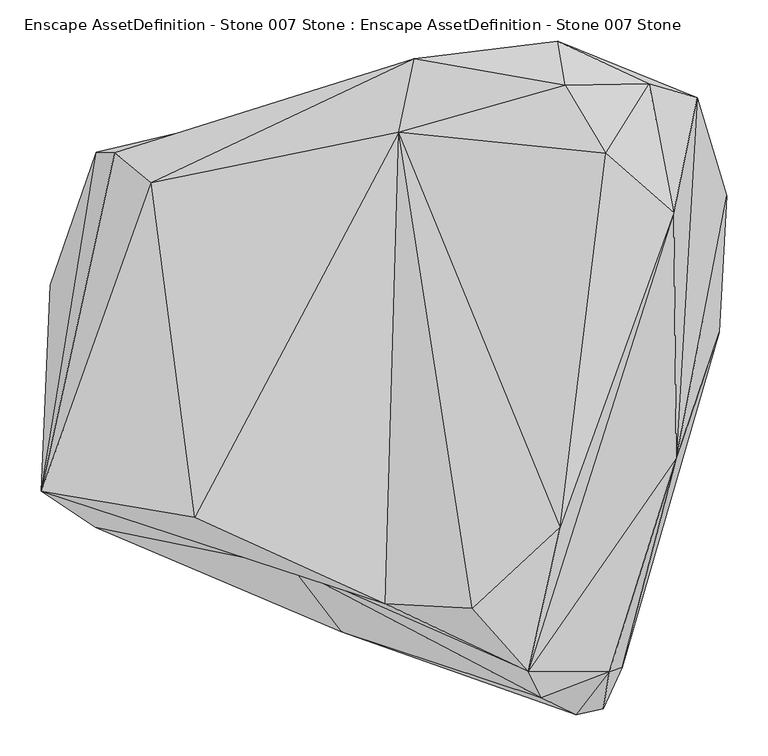
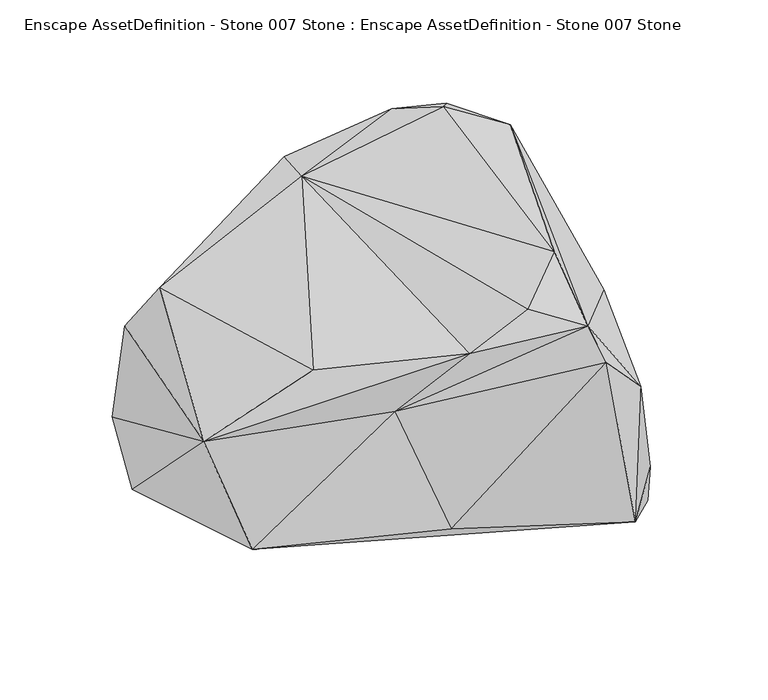
"""IFC4 building model written with IfcOpenShell, lengths in millimetres: geographic element geometry, Enscape AssetDefinition - Stone 007 Stone : Enscape AssetDefinition - Stone 007 Stone."""

import ifcopenshell
import ifcopenshell.guid

model = None  # the IFC model being written
_history = None  # IfcOwnerHistory: only IFC2X3 demands one
_inside = {}  # id of a spatial element -> (the spatial element, [elements in it])
_under = {}  # id of a project, library or spatial element -> (it, [spatial elements below it])
_declared = {}  # id of a project -> (the project, [libraries it declares])
_typed = {}  # id of a type object -> (the type object, [elements of that type])
_made_of = {}  # id of a material, layer set ... -> (it, [elements and type objects made of it])


def new_model(schema):
    """Start an empty IFC model of exactly this schema.

    Asked for "IFC4X3", IfcOpenShell would pick the latest addendum, in which some entities
    have other attributes; the version numbers below select the first issue.
    IFC2X3 requires an IfcOwnerHistory on every rooted entity: one is made here for all.
    """
    global model, _history
    if schema == "IFC4X3":
        model = ifcopenshell.file(schema_version=(4, 3, 0, 0))
    else:
        model = ifcopenshell.file(schema=schema)
    _inside.clear()
    _under.clear()
    _declared.clear()
    _typed.clear()
    _made_of.clear()
    _history = None
    if model.schema == "IFC2X3":
        org = make("IfcOrganization", Name="unknown")
        user = make(
            "IfcPersonAndOrganization",
            ThePerson=make("IfcPerson", FamilyName="unknown"),
            TheOrganization=org,
        )
        app = make(
            "IfcApplication",
            ApplicationDeveloper=org,
            Version="unknown",
            ApplicationFullName="unknown",
            ApplicationIdentifier="unknown",
        )
        _history = make(
            "IfcOwnerHistory",
            OwningUser=user,
            OwningApplication=app,
            ChangeAction="ADDED",
            CreationDate=0,
        )
    return model


def make(cls, **values):
    """One entity of the class cls with the attributes given. An attribute that is None is left unset."""
    return model.create_entity(
        cls, **{name: value for name, value in values.items() if value is not None}
    )


def rooted(cls, **values):
    """An entity with a GlobalId (a new one), such as an element, a storey or a relation."""
    return make(cls, GlobalId=ifcopenshell.guid.new(), OwnerHistory=_history, **values)


def si_unit(unit_type, name, prefix=None):
    """IfcSIUnit, for example si_unit("LENGTHUNIT", "METRE", prefix="MILLI")."""
    return make("IfcSIUnit", UnitType=unit_type, Prefix=prefix, Name=name)


def assignment(units):
    """IfcUnitAssignment: the units of a project."""
    return None if units is None else make("IfcUnitAssignment", Units=units)


def point(xyz):
    """IfcCartesianPoint."""
    return None if xyz is None else make("IfcCartesianPoint", Coordinates=xyz)


def direction(xyz):
    """IfcDirection."""
    return None if xyz is None else make("IfcDirection", DirectionRatios=xyz)


def frame(location, z_axis=None, x_axis=None):
    """IfcAxis2Placement3D, a coordinate frame: its origin and axes. An axis left out is left unset."""
    return make(
        "IfcAxis2Placement3D",
        Location=point(location),
        Axis=direction(z_axis),
        RefDirection=direction(x_axis),
    )


def origin():
    """The frame at (0, 0, 0) with its axes left unset."""
    return frame((0.0, 0.0, 0.0))


def place(relative_to, where):
    """IfcLocalPlacement: puts the frame where relative to a parent placement (None: the world)."""
    return make(
        "IfcLocalPlacement", PlacementRelTo=relative_to, RelativePlacement=where
    )


def context(
    kind, dimensions, precision=None, world=None, true_north=None, identifier=None
):
    """IfcGeometricRepresentationContext, for example the 3D "Model" context."""
    return make(
        "IfcGeometricRepresentationContext",
        ContextIdentifier=identifier,
        ContextType=kind,
        CoordinateSpaceDimension=dimensions,
        Precision=precision,
        WorldCoordinateSystem=world,
        TrueNorth=true_north,
    )


def project(units=None, contexts=None):
    """IfcProject with its units and contexts."""
    return rooted(
        "IfcProject",
        Name="project",
        RepresentationContexts=contexts,
        UnitsInContext=assignment(units),
    )


def spatial(cls, under=None, at=None, **own):
    """A site, building, storey or space (cls), placed at a placement, below another one or the project."""
    s = rooted(cls, ObjectPlacement=at, **own)
    if under is not None:
        _under.setdefault(under.id(), (under, []))[1].append(s)
    return s


def faces_of(points, faces, orient=None, outer=None):
    """IfcFace entities. A face is a list of loops; a loop is a list of indices into points, from 0.

    orient and outer hold one flag for each loop. By default every Orientation is true, the
    first loop of a face is its IfcFaceOuterBound and the others are IfcFaceBound.
    """
    made = []
    for i, loops in enumerate(faces):
        bounds = []
        for j, loop in enumerate(loops):
            is_outer = j == 0 if outer is None else outer[i][j]
            bounds.append(
                make(
                    "IfcFaceOuterBound" if is_outer else "IfcFaceBound",
                    Bound=make("IfcPolyLoop", Polygon=[points[k] for k in loop]),
                    Orientation=True if orient is None else orient[i][j],
                )
            )
        made.append(make("IfcFace", Bounds=bounds))
    return made


def faceted_brep(points, faces, orient=None, outer=None, voids=None):
    """IfcFacetedBrep: a solid bounded by flat faces; with voids (closed shells), ...WithVoids."""
    shared = [point(p) for p in points]
    hull = make("IfcClosedShell", CfsFaces=faces_of(shared, faces, orient, outer))
    if voids is None:
        return make("IfcFacetedBrep", Outer=hull)
    return make(
        "IfcFacetedBrepWithVoids",
        Outer=hull,
        Voids=[
            make(cls, CfsFaces=faces_of(shared, fs, o, b)) for cls, fs, o, b in voids
        ],
    )


def shape(context_of_items, identifier, shape_type, items):
    """IfcShapeRepresentation: the items that make up one representation, for example the "Body"."""
    return make(
        "IfcShapeRepresentation",
        ContextOfItems=context_of_items,
        RepresentationIdentifier=identifier,
        RepresentationType=shape_type,
        Items=items,
    )


def source(mapping_origin, context_of_items, identifier, shape_type, items):
    """IfcRepresentationMap: a shape defined once, which mapped items show again and again."""
    return make(
        "IfcRepresentationMap",
        MappingOrigin=mapping_origin,
        MappedRepresentation=shape(context_of_items, identifier, shape_type, items),
    )


def transform(
    local_origin,
    x_axis=None,
    y_axis=None,
    z_axis=None,
    scale=None,
    scale2=None,
    scale3=None,
    uniform=True,
):
    """IfcCartesianTransformationOperator3D, or its non-uniform kind. x_axis, y_axis, z_axis: its Axis1, 2, 3."""
    if uniform:
        return make(
            "IfcCartesianTransformationOperator3D",
            Axis1=direction(x_axis),
            Axis2=direction(y_axis),
            LocalOrigin=point(local_origin),
            Scale=scale,
            Axis3=direction(z_axis),
        )
    return make(
        "IfcCartesianTransformationOperator3DnonUniform",
        Axis1=direction(x_axis),
        Axis2=direction(y_axis),
        LocalOrigin=point(local_origin),
        Scale=scale,
        Axis3=direction(z_axis),
        Scale2=scale2,
        Scale3=scale3,
    )


def mapped(mapping_source, mapping_target):
    """IfcMappedItem: shows the shape of a source again, moved by a transform."""
    return make(
        "IfcMappedItem", MappingSource=mapping_source, MappingTarget=mapping_target
    )


def made_of(thing, what):
    """Note that an element or type object is made of a material, layer set ...; save() writes the relation."""
    if what is not None:
        _made_of.setdefault(what.id(), (what, []))[1].append(thing)
    return thing


def element(
    cls,
    number,
    at=None,
    inside=None,
    cuts=None,
    type_object=None,
    material=None,
    context=None,
    identifier="Body",
    shape_type=None,
    held_by="IfcProductDefinitionShape",
    body=None,
    shapes=None,
    **own,
):
    """One element of the class cls, such as IfcWall. Its Tag is "e" and its number.

    at: its placement. inside: the storey or other place that contains it. cuts: it is an
    opening in that element (IfcRelVoidsElement). A single representation is given by context,
    identifier, shape_type and body (its items); several are given by shapes. held_by: the class
    of the entity that holds the representations. save() writes the other relations.
    """
    e = rooted(cls, Tag="e%d" % number, ObjectPlacement=at, **own)
    if body is not None:
        shapes = [shape(context, identifier, shape_type, body)]
    if shapes is not None:
        e.Representation = make(held_by, Representations=shapes)
    if inside is not None:
        _inside.setdefault(inside.id(), (inside, []))[1].append(e)
    if cuts is not None:
        rooted(
            "IfcRelVoidsElement", RelatingBuildingElement=cuts, RelatedOpeningElement=e
        )
    if type_object is not None:
        _typed.setdefault(type_object.id(), (type_object, []))[1].append(e)
    return made_of(e, material)


def aggregate(whole, parts):
    """IfcRelAggregates: a whole, such as a stair, and the parts it consists of."""
    return rooted("IfcRelAggregates", RelatingObject=whole, RelatedObjects=parts)


def save(model, path):
    """Write the relations noted so far, then the file.

    IfcRelAggregates (storeys below a building ...), IfcRelContainedInSpatialStructure (elements
    in a storey), IfcRelDefinesByType, IfcRelAssociatesMaterial and IfcRelDeclares: one each for
    every whole, place, type object, material and project.
    """
    for whole, parts in _under.values():
        aggregate(whole, parts)
    for where, things in _inside.values():
        rooted(
            "IfcRelContainedInSpatialStructure",
            RelatedElements=things,
            RelatingStructure=where,
        )
    for kind, things in _typed.values():
        rooted("IfcRelDefinesByType", RelatedObjects=things, RelatingType=kind)
    for what, things in _made_of.values():
        rooted("IfcRelAssociatesMaterial", RelatedObjects=things, RelatingMaterial=what)
    for by, libraries in _declared.values():
        rooted("IfcRelDeclares", RelatingContext=by, RelatedDefinitions=libraries)
    model.write(path)


def enscape_assetdefinition_stone_007_stone_enscape_823d60b0(model_context):
    return source(origin(), model_context, "Body", "Brep", [
        faceted_brep([(224.847436, -174.5665222, 412.6452506), (363.1648719, 207.8361958, 383.7472498), (280.3442776, 280.4059386, 404.5871496), (333.5339725, 364.9718463, 341.812849), (391.9306397, 347.7776051, 246.3645637), (185.9779656, -350.0419855, 385.1563931), (366.1512434, -90.8051431, 237.0504588), (28.6185723, 305.9436381, 339.8826122), (230.8758497, 363.1937504, 367.601186), (117.9578826, -273.6137509, 396.4365423), (12.2159477, -268.3600187, 341.632843), (-272.9106843, 244.3567514, 261.6812289), (-219.8124826, -162.8050506, 326.1500895), (47.5888923, 395.4848349, 317.5778389), (221.7974216, 416.7802036, 318.7632561), (-317.4764216, 280.5779576, 179.1678965), (116.8490648, 389.3291354, 54.4019379), (-406.9549441, -131.0897321, 230.9613675), (-102.0385697, -223.5009223, 240.2436584), (-339.9760723, 281.7066908, 6.0771457), (-395.9980011, 119.5291281, -19.7330713), (-340.9456611, -174.9802381, 20.9592413), (249.5657355, 303.727001, -3.7451368), (418.8278019, 62.5018179, -46.8271337), (300.7983267, -345.4555273, -3.5024884), (244.4850355, -403.0079246, 8.300758), (-41.6648947, -301.9837141, 33.5023664), (284.8978937, -350.8773446, 231.6932976), (277.2813439, -395.7951069, 101.3454273), (427.9370606, 228.6422849, 6.5743756), (202.1468729, -382.6274574, 327.321589), (406.8664312, 288.1915569, 38.3036211)], [[[0, 1, 2]], [[1, 3, 2]], [[3, 1, 4]], [[0, 5, 1]], [[1, 6, 4]], [[5, 6, 1]], [[0, 2, 7]], [[7, 2, 8]], [[2, 3, 8]], [[0, 7, 9]], [[9, 5, 0]], [[9, 7, 10]], [[10, 5, 9]], [[11, 12, 7]], [[7, 12, 10]], [[7, 8, 13]], [[13, 11, 7]], [[8, 3, 14]], [[8, 14, 13]], [[15, 13, 16]], [[14, 16, 13]], [[13, 15, 11]], [[12, 11, 17]], [[11, 15, 17]], [[12, 17, 10]], [[17, 18, 10]], [[18, 5, 10]], [[15, 19, 17]], [[17, 20, 21]], [[18, 17, 21]], [[17, 19, 20]], [[19, 15, 16]], [[19, 22, 23]], [[20, 19, 23]], [[19, 16, 22]], [[23, 24, 20]], [[21, 20, 24]], [[21, 24, 25]], [[26, 18, 21]], [[26, 21, 25]], [[24, 6, 27]], [[23, 6, 24]], [[24, 27, 28]], [[24, 28, 25]], [[23, 29, 6]], [[22, 29, 23]], [[4, 6, 29]], [[27, 6, 5]], [[27, 30, 25]], [[5, 30, 27]], [[27, 25, 28]], [[25, 30, 26]], [[18, 26, 30]], [[5, 18, 30]], [[4, 31, 14]], [[3, 4, 14]], [[31, 4, 29]], [[31, 29, 22]], [[16, 14, 31]], [[16, 31, 22]]]),
    ])


if __name__ == "__main__":
    model = new_model("IFC4")
    model_context = context("Model", 3, world=origin())
    ifc_project = project(units=[si_unit("LENGTHUNIT", "METRE", prefix="MILLI")], contexts=[model_context])
    site = spatial("IfcSite", under=ifc_project)
    building = spatial("IfcBuilding", under=site)
    placement = place(None, origin())
    enscape_assetdefinition_stone_007_stone_enscape_shape = enscape_assetdefinition_stone_007_stone_enscape_823d60b0(model_context)
    element("IfcGeographicElement", 1, ObjectType="Enscape AssetDefinition - Stone 007 Stone : Enscape AssetDefinition - Stone 007 Stone", at=placement, inside=building, context=model_context, shape_type="MappedRepresentation", body=[
        mapped(enscape_assetdefinition_stone_007_stone_enscape_shape, transform((0.0, 0.0, 0.0), x_axis=(1.0, 0.0, 0.0), y_axis=(0.0, 1.0, 0.0), z_axis=(0.0, 0.0, 1.0))),
    ])
    save(model, "model.ifc")

# Revit data of these elements
# Type "Enscape AssetDefinition - Stone 007 Stone : Enscape AssetDefinition - Stone 007 Stone"
#   EnscapeAssetSource = "REMOTE"
#   EnscapeAssetId = "5933aa18-90c0-4cbc-9fcb-b684288696e0"
#   Height = 0.412645 m
#   EnscapeNativeAssetHeight = 0.412645 m
#   Default Elevation = 0
